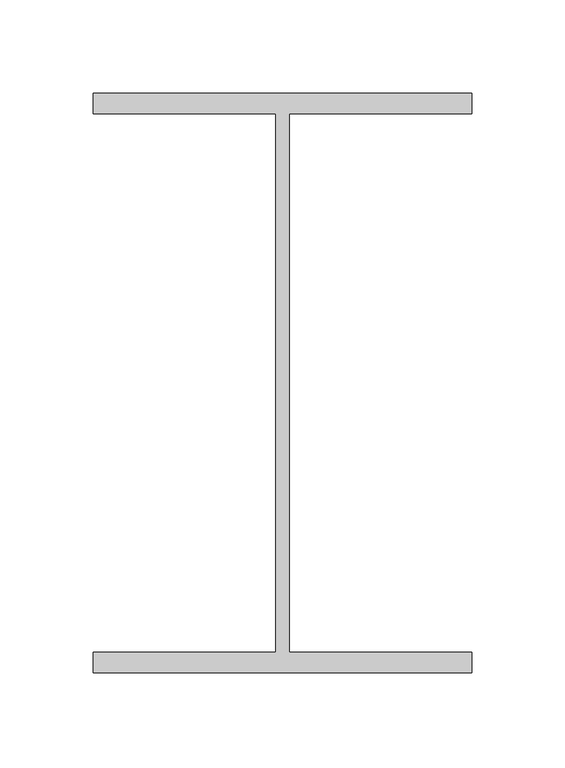
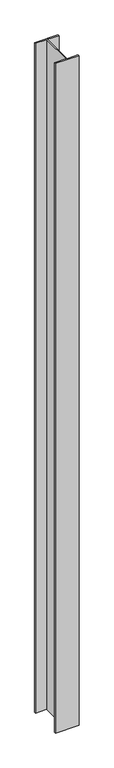
"""IFC4 building model written with IfcOpenShell, lengths in millimetres: proxy geometry, Generic Models 2:Generic Models 2:310765:Generic Models 2:310765 : Generic Models 2:Generic Models 2:310765:83 : Generic Models 2:Generic Models 2:310765:Generic Models 2:310765 : Generic Models 2:Generic Models 2:310765:300385."""

from ifc_helpers import new_model, si_unit, origin, origin_with_axes, place, context, project, spatial, polyline, outline, extrude, source, transform, mapped, element, save


def generic_models_91bb2585(model_context):
    return source(origin(), model_context, "Body", "SweptSolid", [
        extrude(outline(polyline([(579104.5117239, -567621.4913841), (579104.5117239, -567632.5046653), (579006.5828177, -567632.5046653), (579006.5828177, -567921.6281028), (579104.5117239, -567921.6281028), (579104.5117239, -567932.6413841), (578901.2863239, -567932.6413841), (578901.2863239, -567921.6281028), (578999.2406302, -567921.6281028), (578999.2406302, -567632.5046653), (578901.3117239, -567632.5046653), (578901.3117239, -567621.4913841), (579104.5117239, -567621.4913841)])), origin_with_axes(), (0.0, 0.0, 1.0), 6134.1),
    ])


if __name__ == "__main__":
    model = new_model("IFC4")
    model_context = context("Model", 3, world=origin())
    ifc_project = project(units=[si_unit("LENGTHUNIT", "METRE", prefix="MILLI")], contexts=[model_context])
    site = spatial("IfcSite", under=ifc_project)
    building = spatial("IfcBuilding", under=site)
    placement = place(None, origin())
    generic_models_shape = generic_models_91bb2585(model_context)
    element("IfcBuildingElementProxy", 1, Name="Generic Models 2:Generic Models 2:310765:Generic Models 2:310765 : Generic Models 2:Generic Models 2:310765:83 : Generic Models 2:Generic Models 2:310765:Generic Models 2:310765 : Generic Models 2:Generic Models 2:310765:300385", ObjectType="Generic Models 2:Generic Models 2:310765:Generic Models 2:310765 : Generic Models 2:Generic Models 2:310765:83 : Generic Models 2:Generic Models 2:310765:Generic Models 2:310765 : Generic Models 2:Generic Models 2:310765:300385", at=placement, inside=building, context=model_context, shape_type="MappedRepresentation", body=[
        mapped(generic_models_shape, transform((0.0, 0.0, 0.0), x_axis=(1.0, 0.0, 0.0), y_axis=(0.0, 1.0, 0.0), z_axis=(0.0, 0.0, 1.0))),
    ])
    save(model, "model.ifc")

# Revit data of these elements
# Type "Generic Models 2:Generic Models 2:310765:Generic Models 2:310765 : Generic Models 2:Generic Models 2:310765:83 : Generic Models 2:Generic Models 2:310765:Generic Models 2:310765 : Generic Models 2:Generic Models 2:310765:300385"
#   NameOverride = "Generic Models 2:Generic Models 2:310765:Generic Models 2:310765 : Generic Models 2:Generic Models 2:310765:300385"
#   ObjectTypeOverride = "Generic Models 2:310765 : Generic Models 2:Generic Models 2:310765"
#   Reference = "Generic Models 2"
#   Tag = "300385"
# Element 1 (IfcBuildingElementProxy, "Generic Models 2:Generic Models 2:310765:Generic Models 2:310765 : Generic Models 2:Generic Models 2:310765:83 : Generic Models 2:Generic Models 2:310765:Generic Models 2:310765 : Generic Models 2:Generic Models 2:310765:300385")
#   Materials on its faces: "STRUCTURAL STEEL - SEE STRUCT. DWGS"
# Materials
#   "STRUCTURAL STEEL - SEE STRUCT. DWGS": class "Metal", colour RGB 189 187 185, transparency 0, Description = "Structural steel 50ksi", Cost = 0
